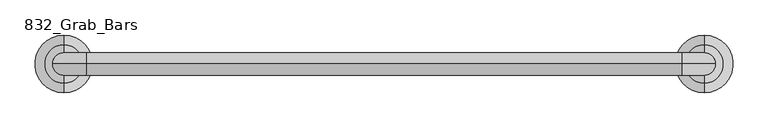
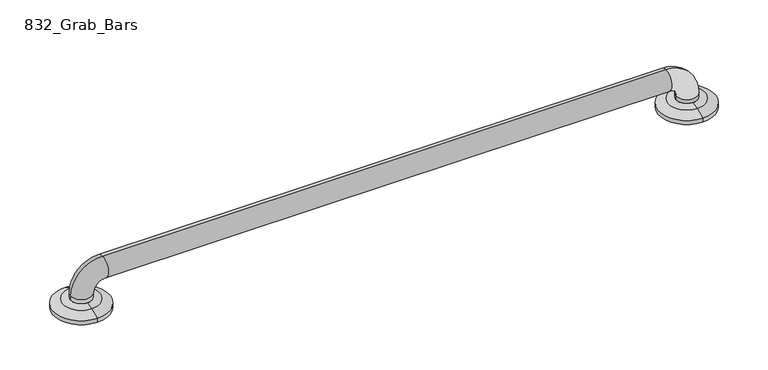
"""IFC4 building model written with IfcOpenShell, lengths in millimetres: proxy geometry, 832_Grab_Bars : 8320-001360."""

import ifcopenshell
import ifcopenshell.guid

model = None  # the IFC model being written
_history = None  # IfcOwnerHistory: only IFC2X3 demands one
_inside = {}  # id of a spatial element -> (the spatial element, [elements in it])
_under = {}  # id of a project, library or spatial element -> (it, [spatial elements below it])
_declared = {}  # id of a project -> (the project, [libraries it declares])
_typed = {}  # id of a type object -> (the type object, [elements of that type])
_made_of = {}  # id of a material, layer set ... -> (it, [elements and type objects made of it])


def new_model(schema):
    """Start an empty IFC model of exactly this schema.

    Asked for "IFC4X3", IfcOpenShell would pick the latest addendum, in which some entities
    have other attributes; the version numbers below select the first issue.
    IFC2X3 requires an IfcOwnerHistory on every rooted entity: one is made here for all.
    """
    global model, _history
    if schema == "IFC4X3":
        model = ifcopenshell.file(schema_version=(4, 3, 0, 0))
    else:
        model = ifcopenshell.file(schema=schema)
    _inside.clear()
    _under.clear()
    _declared.clear()
    _typed.clear()
    _made_of.clear()
    _history = None
    if model.schema == "IFC2X3":
        org = make("IfcOrganization", Name="unknown")
        user = make(
            "IfcPersonAndOrganization",
            ThePerson=make("IfcPerson", FamilyName="unknown"),
            TheOrganization=org,
        )
        app = make(
            "IfcApplication",
            ApplicationDeveloper=org,
            Version="unknown",
            ApplicationFullName="unknown",
            ApplicationIdentifier="unknown",
        )
        _history = make(
            "IfcOwnerHistory",
            OwningUser=user,
            OwningApplication=app,
            ChangeAction="ADDED",
            CreationDate=0,
        )
    return model


def make(cls, **values):
    """One entity of the class cls with the attributes given. An attribute that is None is left unset."""
    return model.create_entity(
        cls, **{name: value for name, value in values.items() if value is not None}
    )


def rooted(cls, **values):
    """An entity with a GlobalId (a new one), such as an element, a storey or a relation."""
    return make(cls, GlobalId=ifcopenshell.guid.new(), OwnerHistory=_history, **values)


def si_unit(unit_type, name, prefix=None):
    """IfcSIUnit, for example si_unit("LENGTHUNIT", "METRE", prefix="MILLI")."""
    return make("IfcSIUnit", UnitType=unit_type, Prefix=prefix, Name=name)


def assignment(units):
    """IfcUnitAssignment: the units of a project."""
    return None if units is None else make("IfcUnitAssignment", Units=units)


def point(xyz):
    """IfcCartesianPoint."""
    return None if xyz is None else make("IfcCartesianPoint", Coordinates=xyz)


def direction(xyz):
    """IfcDirection."""
    return None if xyz is None else make("IfcDirection", DirectionRatios=xyz)


def frame(location, z_axis=None, x_axis=None):
    """IfcAxis2Placement3D, a coordinate frame: its origin and axes. An axis left out is left unset."""
    return make(
        "IfcAxis2Placement3D",
        Location=point(location),
        Axis=direction(z_axis),
        RefDirection=direction(x_axis),
    )


def origin():
    """The frame at (0, 0, 0) with its axes left unset."""
    return frame((0.0, 0.0, 0.0))


def place(relative_to, where):
    """IfcLocalPlacement: puts the frame where relative to a parent placement (None: the world)."""
    return make(
        "IfcLocalPlacement", PlacementRelTo=relative_to, RelativePlacement=where
    )


def context(
    kind, dimensions, precision=None, world=None, true_north=None, identifier=None
):
    """IfcGeometricRepresentationContext, for example the 3D "Model" context."""
    return make(
        "IfcGeometricRepresentationContext",
        ContextIdentifier=identifier,
        ContextType=kind,
        CoordinateSpaceDimension=dimensions,
        Precision=precision,
        WorldCoordinateSystem=world,
        TrueNorth=true_north,
    )


def project(units=None, contexts=None):
    """IfcProject with its units and contexts."""
    return rooted(
        "IfcProject",
        Name="project",
        RepresentationContexts=contexts,
        UnitsInContext=assignment(units),
    )


def spatial(cls, under=None, at=None, **own):
    """A site, building, storey or space (cls), placed at a placement, below another one or the project."""
    s = rooted(cls, ObjectPlacement=at, **own)
    if under is not None:
        _under.setdefault(under.id(), (under, []))[1].append(s)
    return s


def polyline(points):
    """IfcPolyline through the points."""
    return make("IfcPolyline", Points=[point(p) for p in points])


def circle_curve(where, radius):
    """IfcCircle in the frame where."""
    return make("IfcCircle", Position=where, Radius=radius)


def ellipse_curve(where, semi_axis1, semi_axis2):
    """IfcEllipse in the frame where."""
    return make(
        "IfcEllipse", Position=where, SemiAxis1=semi_axis1, SemiAxis2=semi_axis2
    )


def trimmed(basis, trim1, trim2, sense, master):
    """IfcTrimmedCurve: the piece of a basis curve between two trims."""
    return make(
        "IfcTrimmedCurve",
        BasisCurve=basis,
        Trim1=trim1,
        Trim2=trim2,
        SenseAgreement=sense,
        MasterRepresentation=master,
    )


def shape(context_of_items, identifier, shape_type, items):
    """IfcShapeRepresentation: the items that make up one representation, for example the "Body"."""
    return make(
        "IfcShapeRepresentation",
        ContextOfItems=context_of_items,
        RepresentationIdentifier=identifier,
        RepresentationType=shape_type,
        Items=items,
    )


def source(mapping_origin, context_of_items, identifier, shape_type, items):
    """IfcRepresentationMap: a shape defined once, which mapped items show again and again."""
    return make(
        "IfcRepresentationMap",
        MappingOrigin=mapping_origin,
        MappedRepresentation=shape(context_of_items, identifier, shape_type, items),
    )


def transform(
    local_origin,
    x_axis=None,
    y_axis=None,
    z_axis=None,
    scale=None,
    scale2=None,
    scale3=None,
    uniform=True,
):
    """IfcCartesianTransformationOperator3D, or its non-uniform kind. x_axis, y_axis, z_axis: its Axis1, 2, 3."""
    if uniform:
        return make(
            "IfcCartesianTransformationOperator3D",
            Axis1=direction(x_axis),
            Axis2=direction(y_axis),
            LocalOrigin=point(local_origin),
            Scale=scale,
            Axis3=direction(z_axis),
        )
    return make(
        "IfcCartesianTransformationOperator3DnonUniform",
        Axis1=direction(x_axis),
        Axis2=direction(y_axis),
        LocalOrigin=point(local_origin),
        Scale=scale,
        Axis3=direction(z_axis),
        Scale2=scale2,
        Scale3=scale3,
    )


def mapped(mapping_source, mapping_target):
    """IfcMappedItem: shows the shape of a source again, moved by a transform."""
    return make(
        "IfcMappedItem", MappingSource=mapping_source, MappingTarget=mapping_target
    )


def made_of(thing, what):
    """Note that an element or type object is made of a material, layer set ...; save() writes the relation."""
    if what is not None:
        _made_of.setdefault(what.id(), (what, []))[1].append(thing)
    return thing


def element(
    cls,
    number,
    at=None,
    inside=None,
    cuts=None,
    type_object=None,
    material=None,
    context=None,
    identifier="Body",
    shape_type=None,
    held_by="IfcProductDefinitionShape",
    body=None,
    shapes=None,
    **own,
):
    """One element of the class cls, such as IfcWall. Its Tag is "e" and its number.

    at: its placement. inside: the storey or other place that contains it. cuts: it is an
    opening in that element (IfcRelVoidsElement). A single representation is given by context,
    identifier, shape_type and body (its items); several are given by shapes. held_by: the class
    of the entity that holds the representations. save() writes the other relations.
    """
    e = rooted(cls, Tag="e%d" % number, ObjectPlacement=at, **own)
    if body is not None:
        shapes = [shape(context, identifier, shape_type, body)]
    if shapes is not None:
        e.Representation = make(held_by, Representations=shapes)
    if inside is not None:
        _inside.setdefault(inside.id(), (inside, []))[1].append(e)
    if cuts is not None:
        rooted(
            "IfcRelVoidsElement", RelatingBuildingElement=cuts, RelatedOpeningElement=e
        )
    if type_object is not None:
        _typed.setdefault(type_object.id(), (type_object, []))[1].append(e)
    return made_of(e, material)


def aggregate(whole, parts):
    """IfcRelAggregates: a whole, such as a stair, and the parts it consists of."""
    return rooted("IfcRelAggregates", RelatingObject=whole, RelatedObjects=parts)


def save(model, path):
    """Write the relations noted so far, then the file.

    IfcRelAggregates (storeys below a building ...), IfcRelContainedInSpatialStructure (elements
    in a storey), IfcRelDefinesByType, IfcRelAssociatesMaterial and IfcRelDeclares: one each for
    every whole, place, type object, material and project.
    """
    for whole, parts in _under.values():
        aggregate(whole, parts)
    for where, things in _inside.values():
        rooted(
            "IfcRelContainedInSpatialStructure",
            RelatedElements=things,
            RelatingStructure=where,
        )
    for kind, things in _typed.values():
        rooted("IfcRelDefinesByType", RelatedObjects=things, RelatingType=kind)
    for what, things in _made_of.values():
        rooted("IfcRelAssociatesMaterial", RelatedObjects=things, RelatingMaterial=what)
    for by, libraries in _declared.values():
        rooted("IfcRelDeclares", RelatingContext=by, RelatedDefinitions=libraries)
    model.write(path)


def plane_surface(at):
    """IfcPlane: the flat surface through the origin of the frame at, square to its z axis."""
    return make("IfcPlane", Position=at)


def cylinder_surface(at, radius):
    """IfcCylindricalSurface: all points at the distance radius from the z axis of the frame at."""
    return make("IfcCylindricalSurface", Position=at, Radius=radius)


def revolved_surface(curve, axis_point, axis_direction):
    """IfcSurfaceOfRevolution: the curve turned about the line through axis_point along axis_direction."""
    return make(
        "IfcSurfaceOfRevolution",
        SweptCurve=make("IfcArbitraryOpenProfileDef", ProfileType="CURVE", Curve=curve),
        AxisPosition=make("IfcAxis1Placement", Location=point(axis_point), Axis=direction(axis_direction)),
    )


def advanced_brep(points, edges, surfaces, faces):
    """IfcAdvancedBrep: a solid bounded by faces that lie on surfaces and meet in shared edges.

    An edge is (start, end): straight between two places in points (the first is 0);
    or (start, end, curve); or (start, end, curve, False) where it runs against its curve.
    A face is (place in surfaces, loops), or (place, loops, False) where it looks against
    its surface's normal. A loop lists edges by number (the first is 1), with a minus sign
    where the edge is run from its end to its start. The first loop is the outer one.
    """
    corners = [point(p) for p in points]
    vertices = [make("IfcVertexPoint", VertexGeometry=c) for c in corners]
    made = []
    for start, end, *more in edges:
        made.append(
            make(
                "IfcEdgeCurve",
                EdgeStart=vertices[start],
                EdgeEnd=vertices[end],
                EdgeGeometry=more[0] if more else make("IfcPolyline", Points=[corners[start], corners[end]]),
                SameSense=more[1] if len(more) > 1 else True,
            )
        )
    hull = []
    for where, loops, *sense in faces:
        bounds = []
        for j, loop in enumerate(loops):
            ring = [make("IfcOrientedEdge", EdgeElement=made[abs(k) - 1], Orientation=k > 0) for k in loop]
            bounds.append(
                make(
                    "IfcFaceOuterBound" if j == 0 else "IfcFaceBound",
                    Bound=make("IfcEdgeLoop", EdgeList=ring),
                    Orientation=True,
                )
            )
        hull.append(make("IfcAdvancedFace", Bounds=bounds, FaceSurface=surfaces[where], SameSense=sense[0] if sense else True))
    return make("IfcAdvancedBrep", Outer=make("IfcClosedShell", CfsFaces=hull))


def proxy_832_grab_bars_3fec91fc(model_context):
    return source(origin(), model_context, "Body", "AdvancedBrep", [
        advanced_brep(
        [(-363.5375, 564.1630987, 13.1934507), (-363.5375, 577.85, 6.35), (-363.5375, 495.3, 6.35), (-363.5375, 508.9869013, 13.1934507), (-363.5375, 520.3461266, 15.875), (-363.5375, 552.8038734, 15.875), (-363.5375, 520.7, 15.875), (-379.4125, 536.575, 15.875), (-363.5375, 552.45, 15.875), (-347.6625, 536.575, 15.875), (-363.5375, 577.85, 0.0), (-363.5375, 552.45, 0.0), (-363.5375, 536.575, 0.0), (-363.5375, 520.7, 0.0), (-363.5375, 495.3, 0.0), (550.8625, 564.2276895, 13.1934507), (550.8625, 577.9145908, 6.35), (550.8625, 495.3645908, 6.35), (550.8625, 509.0514921, 13.1934507), (550.8625, 520.4107174, 15.875), (550.8625, 552.8684641, 15.875), (550.8625, 520.7, 15.875), (534.9875, 536.575, 15.875), (550.8625, 552.45, 15.875), (566.7375, 536.575, 15.875), (550.8625, 577.9145908, 0.0), (550.8625, 552.45, 0.0), (550.8625, 536.6395908, 0.0), (550.8625, 520.7, 0.0), (550.8625, 495.3645908, 0.0), (-379.4125, 536.575, 22.225), (-347.6625, 536.575, 22.225), (-331.7875, 536.575, 38.1), (-331.7875, 536.575, 69.85), (519.1125, 536.575, 38.1), (519.1125, 536.575, 69.85), (534.9875, 536.575, 22.225), (566.7375, 536.575, 22.225)],
        [
            (0, 1),
            (1, 2, circle_curve(frame((-363.5375, 536.575, 6.35), z_axis=(0.0, 0.0, 1.0), x_axis=(0.0, -1.0, 0.0)), 41.275)),
            (2, 3),
            (3, 0, circle_curve(frame((-363.5375, 536.575, 13.1934507), z_axis=(0.0, 0.0, -1.0), x_axis=(0.0, -1.0, 0.0)), 27.5880987)),
            (2, 1, circle_curve(frame((-363.5375, 536.575, 6.35), z_axis=(0.0, 0.0, 1.0), x_axis=(0.0, -1.0, 0.0)), 41.275)),
            (0, 3, circle_curve(frame((-363.5375, 536.575, 13.1934507), z_axis=(0.0, 0.0, -1.0), x_axis=(0.0, -1.0, 0.0)), 27.5880987)),
            (3, 4, circle_curve(frame((-363.5375, 520.3461266, -9.525), z_axis=(-1.0, 0.0, 0.0), x_axis=(0.0, 0.0, -1.0)), 25.4)),
            (4, 5, circle_curve(frame((-363.5375, 536.575, 15.875), z_axis=(0.0, 0.0, -1.0), x_axis=(0.0, -1.0, 0.0)), 16.2288734)),
            (5, 0, circle_curve(frame((-363.5375, 552.8038734, -9.525), z_axis=(-1.0, 0.0, 0.0), x_axis=(0.0, 0.0, -1.0)), 25.4)),
            (5, 4, circle_curve(frame((-363.5375, 536.575, 15.875), z_axis=(0.0, 0.0, -1.0), x_axis=(0.0, -1.0, 0.0)), 16.2288734)),
            (4, 6),
            (6, 7, circle_curve(frame((-363.5375, 536.575, 15.875), z_axis=(0.0, 0.0, -1.0), x_axis=(1.0, 0.0, 0.0)), 15.875)),
            (7, 8, circle_curve(frame((-363.5375, 536.575, 15.875), z_axis=(0.0, 0.0, -1.0), x_axis=(1.0, 0.0, 0.0)), 15.875)),
            (8, 5),
            (8, 9, circle_curve(frame((-363.5375, 536.575, 15.875), z_axis=(0.0, 0.0, -1.0), x_axis=(1.0, 0.0, 0.0)), 15.875)),
            (9, 6, circle_curve(frame((-363.5375, 536.575, 15.875), z_axis=(0.0, 0.0, -1.0), x_axis=(1.0, 0.0, 0.0)), 15.875)),
            (10, 11),
            (11, 12),
            (12, 13),
            (13, 14),
            (14, 10, circle_curve(frame((-363.5375, 536.575, 0.0), z_axis=(0.0, 0.0, -1.0), x_axis=(0.0, -1.0, 0.0)), 41.275)),
            (10, 14, circle_curve(frame((-363.5375, 536.575, 0.0), z_axis=(0.0, 0.0, -1.0), x_axis=(0.0, -1.0, 0.0)), 41.275)),
            (1, 10),
            (14, 2),
            (15, 16),
            (16, 17, circle_curve(frame((550.8625, 536.6395908, 6.35), z_axis=(0.0, 0.0, 1.0), x_axis=(0.0, -1.0, 0.0)), 41.275)),
            (17, 18),
            (18, 15, circle_curve(frame((550.8625, 536.6395908, 13.1934507), z_axis=(0.0, 0.0, -1.0), x_axis=(0.0, -1.0, 0.0)), 27.5880987)),
            (17, 16, circle_curve(frame((550.8625, 536.6395908, 6.35), z_axis=(0.0, 0.0, 1.0), x_axis=(0.0, -1.0, 0.0)), 41.275)),
            (15, 18, circle_curve(frame((550.8625, 536.6395908, 13.1934507), z_axis=(0.0, 0.0, -1.0), x_axis=(0.0, -1.0, 0.0)), 27.5880987)),
            (18, 19, circle_curve(frame((550.8625, 520.4107174, -9.525), z_axis=(-1.0, 0.0, 0.0), x_axis=(0.0, 0.0, -1.0)), 25.4)),
            (19, 20, circle_curve(frame((550.8625, 536.6395908, 15.875), z_axis=(0.0, 0.0, -1.0), x_axis=(0.0, -1.0, 0.0)), 16.2288734)),
            (20, 15, circle_curve(frame((550.8625, 552.8684641, -9.525), z_axis=(-1.0, 0.0, 0.0), x_axis=(0.0, 0.0, -1.0)), 25.4)),
            (20, 19, circle_curve(frame((550.8625, 536.6395908, 15.875), z_axis=(0.0, 0.0, -1.0), x_axis=(0.0, -1.0, 0.0)), 16.2288734)),
            (19, 21),
            (21, 22, circle_curve(frame((550.8625, 536.575, 15.875), z_axis=(0.0, 0.0, -1.0), x_axis=(-1.0, 0.0, 0.0)), 15.875)),
            (22, 23, circle_curve(frame((550.8625, 536.575, 15.875), z_axis=(0.0, 0.0, -1.0), x_axis=(-1.0, 0.0, 0.0)), 15.875)),
            (23, 20),
            (23, 24, circle_curve(frame((550.8625, 536.575, 15.875), z_axis=(0.0, 0.0, -1.0), x_axis=(-1.0, 0.0, 0.0)), 15.875)),
            (24, 21, circle_curve(frame((550.8625, 536.575, 15.875), z_axis=(0.0, 0.0, -1.0), x_axis=(-1.0, 0.0, 0.0)), 15.875)),
            (25, 26),
            (26, 27),
            (27, 28),
            (28, 29),
            (29, 25, circle_curve(frame((550.8625, 536.6395908, 0.0), z_axis=(0.0, 0.0, -1.0), x_axis=(0.0, -1.0, 0.0)), 41.275)),
            (25, 29, circle_curve(frame((550.8625, 536.6395908, 0.0), z_axis=(0.0, 0.0, -1.0), x_axis=(0.0, -1.0, 0.0)), 41.275)),
            (16, 25),
            (29, 17),
            (30, 7),
            (9, 31),
            (31, 30, circle_curve(frame((-363.5375, 536.575, 22.225), z_axis=(0.0, 0.0, -1.0), x_axis=(1.0, 0.0, 0.0)), 15.875)),
            (30, 31, circle_curve(frame((-363.5375, 536.575, 22.225), z_axis=(0.0, 0.0, -1.0), x_axis=(1.0, 0.0, 0.0)), 15.875)),
            (31, 32, circle_curve(frame((-331.7875, 536.575, 22.225), z_axis=(0.0, 1.0, 0.0), x_axis=(-1.0, 0.0, 0.0)), 15.875)),
            (32, 33, circle_curve(frame((-331.7875, 536.575, 53.975), z_axis=(-1.0, 0.0, 0.0), x_axis=(0.0, 0.0, -1.0)), 15.875)),
            (33, 30, circle_curve(frame((-331.7875, 536.575, 22.225), z_axis=(0.0, -1.0, 0.0), x_axis=(-1.0, 0.0, 0.0)), 47.625)),
            (33, 32, circle_curve(frame((-331.7875, 536.575, 53.975), z_axis=(-1.0, 0.0, 0.0), x_axis=(0.0, 0.0, -1.0)), 15.875)),
            (32, 34),
            (34, 35, circle_curve(frame((519.1125, 536.575, 53.975), z_axis=(-1.0, 0.0, 0.0), x_axis=(0.0, 0.0, -1.0)), 15.875)),
            (35, 33),
            (35, 34, circle_curve(frame((519.1125, 536.575, 53.975), z_axis=(-1.0, 0.0, 0.0), x_axis=(0.0, 0.0, -1.0)), 15.875)),
            (34, 36, circle_curve(frame((519.1125, 536.575, 22.225), z_axis=(0.0, 1.0, 0.0), x_axis=(0.0, 0.0, 1.0)), 15.875)),
            (36, 37, circle_curve(frame((550.8625, 536.575, 22.225), z_axis=(0.0, 0.0, 1.0), x_axis=(-1.0, 0.0, 0.0)), 15.875)),
            (37, 35, circle_curve(frame((519.1125, 536.575, 22.225), z_axis=(0.0, -1.0, 0.0), x_axis=(0.0, 0.0, 1.0)), 47.625)),
            (37, 36, circle_curve(frame((550.8625, 536.575, 22.225), z_axis=(0.0, 0.0, 1.0), x_axis=(-1.0, 0.0, 0.0)), 15.875)),
            (36, 22),
            (24, 37),
        ],
        [
            revolved_surface(polyline([(-363.5375, 495.3, 6.35), (-363.5375, 508.9869013, 13.1934507)]), (-363.5375, 536.575, 31.75), (0.0, 0.0, 1.0)),
            revolved_surface(trimmed(ellipse_curve(frame((-363.5375, 520.3461266, -9.525), z_axis=(-1.0, 0.0, 0.0), x_axis=(0.0, 0.0, -1.0)), 25.4, 25.4), [point((-363.5375, 508.9869013, 13.1934507))], [point((-363.5375, 520.3461266, 15.875))], True, "CARTESIAN"), (-363.5375, 536.575, 31.75), (0.0, 0.0, 1.0)),
            plane_surface(frame((-363.5375, 536.575, 15.875), z_axis=(0.0, 0.0, 1.0), x_axis=(0.0, -1.0, 0.0))),
            plane_surface(frame((-363.5375, 536.575, 0.0), z_axis=(0.0, 0.0, -1.0), x_axis=(0.0, -1.0, 0.0))),
            cylinder_surface(frame((-363.5375, 536.575, 31.75), z_axis=(0.0, 0.0, 1.0), x_axis=(0.0, -1.0, 0.0)), 41.275),
            revolved_surface(polyline([(550.8625, 495.3645908, 6.35), (550.8625, 509.0514921, 13.1934507)]), (550.8625, 536.6395908, 31.75), (0.0, 0.0, 1.0)),
            revolved_surface(trimmed(ellipse_curve(frame((550.8625, 520.4107174, -9.525), z_axis=(-1.0, 0.0, 0.0), x_axis=(0.0, 0.0, -1.0)), 25.4, 25.4), [point((550.8625, 509.0514921, 13.1934507))], [point((550.8625, 520.4107174, 15.875))], True, "CARTESIAN"), (550.8625, 536.6395908, 31.75), (0.0, 0.0, 1.0)),
            plane_surface(frame((550.8625, 536.6395908, 15.875), z_axis=(0.0, 0.0, 1.0), x_axis=(0.0, -1.0, 0.0))),
            plane_surface(frame((550.8625, 536.6395908, 0.0), z_axis=(0.0, 0.0, -1.0), x_axis=(0.0, -1.0, 0.0))),
            cylinder_surface(frame((550.8625, 536.6395908, 31.75), z_axis=(0.0, 0.0, 1.0), x_axis=(0.0, -1.0, 0.0)), 41.275),
            cylinder_surface(frame((-363.5375, 536.575, 0.0), z_axis=(0.0, 0.0, -1.0), x_axis=(1.0, 0.0, 0.0)), 15.875),
            revolved_surface(trimmed(ellipse_curve(frame((-363.5375, 536.575, 22.225), z_axis=(0.0, 0.0, 1.0), x_axis=(1.0, 0.0, 0.0)), 15.875, 15.875), [point((-379.4125, 536.575, 22.225))], [point((-347.6625, 536.575, 22.225))], True, "CARTESIAN"), (-331.7875, 536.575, 22.225), (0.0, -1.0, 0.0)),
            revolved_surface(trimmed(ellipse_curve(frame((-363.5375, 536.575, 22.225), z_axis=(0.0, 0.0, 1.0), x_axis=(1.0, 0.0, 0.0)), 15.875, 15.875), [point((-347.6625, 536.575, 22.225))], [point((-379.4125, 536.575, 22.225))], True, "CARTESIAN"), (-331.7875, 536.575, 22.225), (0.0, -1.0, 0.0)),
            cylinder_surface(frame((-331.7875, 536.575, 53.975), z_axis=(-1.0, 0.0, 0.0), x_axis=(0.0, 0.0, -1.0)), 15.875),
            revolved_surface(trimmed(ellipse_curve(frame((519.1125, 536.575, 53.975), z_axis=(1.0, 0.0, 0.0), x_axis=(0.0, 0.0, -1.0)), 15.875, 15.875), [point((519.1125, 536.575, 69.85))], [point((519.1125, 536.575, 38.1))], True, "CARTESIAN"), (519.1125, 536.575, 22.225), (0.0, -1.0, 0.0)),
            revolved_surface(trimmed(ellipse_curve(frame((519.1125, 536.575, 53.975), z_axis=(1.0, 0.0, 0.0), x_axis=(0.0, 0.0, -1.0)), 15.875, 15.875), [point((519.1125, 536.575, 38.1))], [point((519.1125, 536.575, 69.85))], True, "CARTESIAN"), (519.1125, 536.575, 22.225), (0.0, -1.0, 0.0)),
            cylinder_surface(frame((550.8625, 536.575, 22.225), z_axis=(0.0, 0.0, 1.0), x_axis=(-1.0, 0.0, 0.0)), 15.875),
        ],
        [
            (0, [[1, 2, 3, 4]]),
            (0, [[5, -1, 6, -3]]),
            (1, [[7, 8, 9, -4]]),
            (1, [[-9, 10, -7, -6]]),
            (2, [[11, 12, 13, 14, -8]]),
            (2, [[-14, 15, 16, -11, -10]]),
            (3, [[17, 18, 19, 20, 21]]),
            (3, [[-20, -19, -18, -17, 22]]),
            (4, [[23, -21, 24, -2]]),
            (4, [[-24, -22, -23, -5]]),
            (5, [[25, 26, 27, 28]]),
            (5, [[29, -25, 30, -27]]),
            (6, [[31, 32, 33, -28]]),
            (6, [[-33, 34, -31, -30]]),
            (7, [[35, 36, 37, 38, -32]]),
            (7, [[-38, 39, 40, -35, -34]]),
            (8, [[41, 42, 43, 44, 45]]),
            (8, [[-44, -43, -42, -41, 46]]),
            (9, [[47, -45, 48, -26]]),
            (9, [[-48, -46, -47, -29]]),
            (10, [[49, -12, -16, 50, 51]]),
            (10, [[-50, -15, -13, -49, 52]]),
            (11, [[53, 54, 55, -51]]),
            (12, [[-55, 56, -53, -52]]),
            (13, [[57, 58, 59, -54]]),
            (13, [[-59, 60, -57, -56]]),
            (14, [[61, 62, 63, -58]]),
            (15, [[-63, 64, -61, -60]]),
            (16, [[65, -36, -40, 66, -62]]),
            (16, [[-66, -39, -37, -65, -64]]),
        ],
    ),
    ])


if __name__ == "__main__":
    model = new_model("IFC4")
    model_context = context("Model", 3, world=origin())
    ifc_project = project(units=[si_unit("LENGTHUNIT", "METRE", prefix="MILLI")], contexts=[model_context])
    site = spatial("IfcSite", under=ifc_project)
    building = spatial("IfcBuilding", under=site)
    placement = place(None, origin())
    proxy_832_grab_bars_shape = proxy_832_grab_bars_3fec91fc(model_context)
    element("IfcBuildingElementProxy", 1, Name="832_Grab_Bars : 8320-001360", ObjectType="832_Grab_Bars : 8320-001360", at=placement, inside=building, context=model_context, shape_type="MappedRepresentation", body=[
        mapped(proxy_832_grab_bars_shape, transform((0.0, 0.0, 0.0), x_axis=(1.0, 0.0, 0.0), y_axis=(0.0, 1.0, 0.0), z_axis=(0.0, 0.0, 1.0))),
    ])
    save(model, "model.ifc")

# Revit data of these elements
# Type "832_Grab_Bars : 8320-001360"
#   Warranty Information = "Complete unit, one (1) year"
#   Version = "1.0"
#   Technical Data = "http://www.bradleycorp.com/products/techdata/8820.pdf"
#   URL = "www.bradleycorp.com"
#   Type Comments = "All grab bar configurations are specified using centerline to centerline dimensions."
#   OmniClass Title = ""
#   Modeling Code = ""
#   Model = "8320-001360"
#   Material Note = "FLANGES - 13GA., ESCUTCHEONS - 22GA., TUBING - 18GA."
#   MasterFormat Section Title = ""
#   Manufacturer = "Bradley Corporation"
#   LEED Credit = ""
#   Instructions [instance default] = "This is a face mounted fixture."
#   Industry Standards = "ANSI Standard A117.1, ADA, ABA, ADAAG, UFAS"
#   Fire Rating = "None"
#   Description = "Grab Bars"
#   Copyright = "This Model Data is Property of Bradley Corporation"
#   Complies to NAFTA = "Yes"
#   Complies To Buy American Act = "Yes"
#   Assembly Code = "C1030200"
#   ADA Compliant = "Yes"
#   Radius = 15.875 mm
#   Percentage of Recycled Content = 64.64
#   Overall Length = 996.95 mm
#   OmniClass Code = 0
#   MasterFormat Section Number = 0
#   Length = 914.4 mm
#   Diameter = 31.75 mm
#   Default Elevation = 838.2 mm
#   Material and Finish = Bradley Corp Stainless Steel - Satin
# Element 1 (IfcBuildingElementProxy, "832_Grab_Bars : 8320-001360")
#   Materials on its faces: "Bradley Corp Stainless Steel - Satin"
# Materials
#   "Bradley Corp Stainless Steel - Satin": class "Metal", colour RGB 189 187 185, transparency 0, Manufacturer = "Bradley Corporation", URL = "www.bradleycorp.com", Description = "Stainless Steel - Satin Finish", Cost = 0
